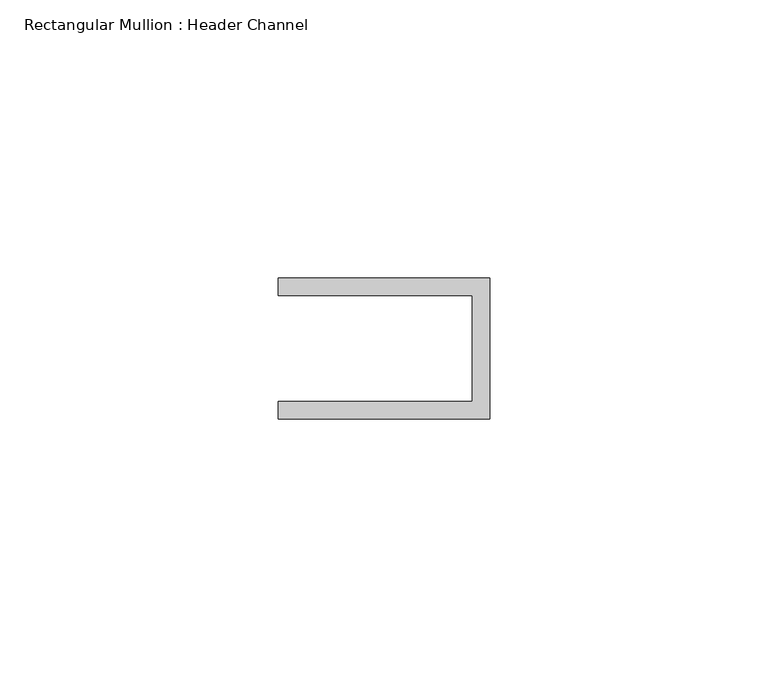
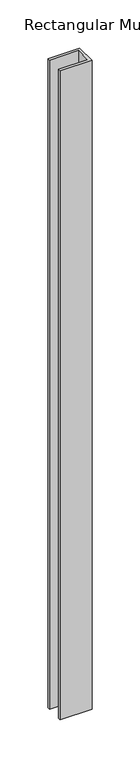
"""IFC4 building model written with IfcOpenShell, lengths in millimetres: member geometry, Rectangular Mullion : Header Channel."""

from ifc_helpers import new_model, si_unit, frame, origin, place, context, project, spatial, polyline, outline, extrude, source, transform, mapped, element, save


def rectangular_mullion_header_channel_3dc9c4af(model_context):
    return source(origin(), model_context, "Body", "SweptSolid", [
        extrude(outline(polyline([(0.0, -12.7), (-38.1, -12.7), (-38.1, -9.525), (-3.175, -9.525), (-3.175, 9.525), (-38.1, 9.525), (-38.1, 12.7), (0.0, 12.7), (0.0, -12.7)])), frame((0.0, 0.0, -823.9125), z_axis=(0.0, 0.0, 1.0), x_axis=(1.0, 0.0, 0.0)), (0.0, 0.0, 1.0), 823.9125),
    ])


if __name__ == "__main__":
    model = new_model("IFC4")
    model_context = context("Model", 3, world=origin())
    ifc_project = project(units=[si_unit("LENGTHUNIT", "METRE", prefix="MILLI")], contexts=[model_context])
    site = spatial("IfcSite", under=ifc_project)
    building = spatial("IfcBuilding", under=site)
    placement = place(None, origin())
    rectangular_mullion_header_channel_shape = rectangular_mullion_header_channel_3dc9c4af(model_context)
    element("IfcMember", 1, ObjectType="Rectangular Mullion : Header Channel", at=placement, inside=building, context=model_context, shape_type="MappedRepresentation", body=[
        mapped(rectangular_mullion_header_channel_shape, transform((0.0, 0.0, 0.0), x_axis=(1.0, 0.0, 0.0), y_axis=(0.0, 1.0, 0.0), z_axis=(0.0, 0.0, 1.0))),
    ])
    save(model, "model.ifc")

# Revit data of these elements
# Type "Rectangular Mullion : Header Channel"
#   built-in parameter 1007322 = 0.0833333 (stored number, unit not read)
#   built-in parameter 1007321 = -0.03125 (stored number, unit not read)
#   built-in parameter 1007320 = 0.0416667 (stored number, unit not read)
# Element 1 (IfcMember, "Rectangular Mullion : Header Channel")
#   Materials on its faces: "ALUM"
# Materials
#   "ALUM": class "Generic", colour RGB 157 157 157, transparency 0, Cost = 0
